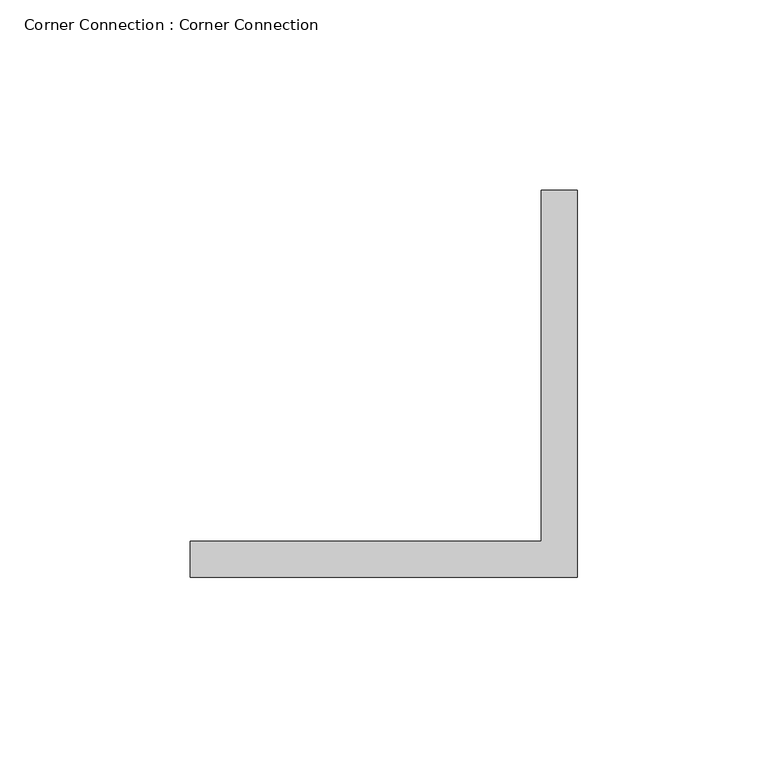
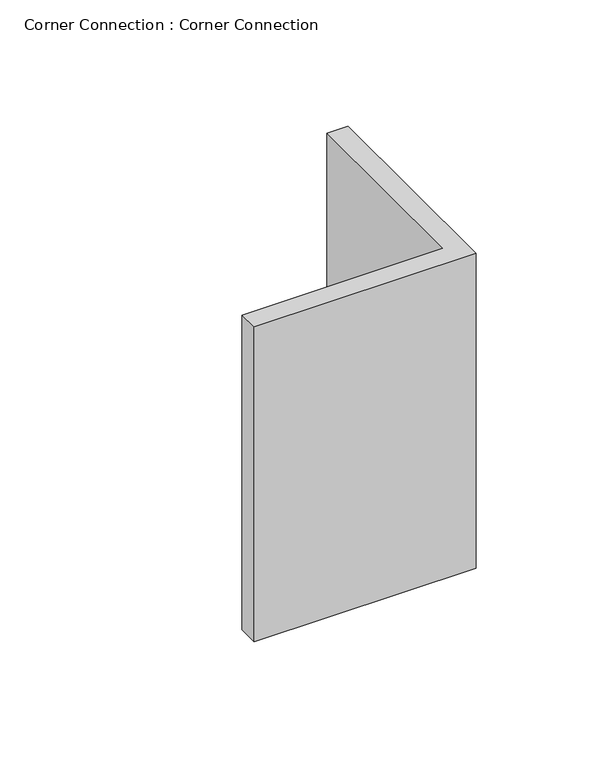
"""IFC4 building model written with IfcOpenShell, lengths in millimetres: fastener geometry, Corner Connection : Corner Connection."""

import ifcopenshell
import ifcopenshell.guid

model = None  # the IFC model being written
_history = None  # IfcOwnerHistory: only IFC2X3 demands one
_inside = {}  # id of a spatial element -> (the spatial element, [elements in it])
_under = {}  # id of a project, library or spatial element -> (it, [spatial elements below it])
_declared = {}  # id of a project -> (the project, [libraries it declares])
_typed = {}  # id of a type object -> (the type object, [elements of that type])
_made_of = {}  # id of a material, layer set ... -> (it, [elements and type objects made of it])


def new_model(schema):
    """Start an empty IFC model of exactly this schema.

    Asked for "IFC4X3", IfcOpenShell would pick the latest addendum, in which some entities
    have other attributes; the version numbers below select the first issue.
    IFC2X3 requires an IfcOwnerHistory on every rooted entity: one is made here for all.
    """
    global model, _history
    if schema == "IFC4X3":
        model = ifcopenshell.file(schema_version=(4, 3, 0, 0))
    else:
        model = ifcopenshell.file(schema=schema)
    _inside.clear()
    _under.clear()
    _declared.clear()
    _typed.clear()
    _made_of.clear()
    _history = None
    if model.schema == "IFC2X3":
        org = make("IfcOrganization", Name="unknown")
        user = make(
            "IfcPersonAndOrganization",
            ThePerson=make("IfcPerson", FamilyName="unknown"),
            TheOrganization=org,
        )
        app = make(
            "IfcApplication",
            ApplicationDeveloper=org,
            Version="unknown",
            ApplicationFullName="unknown",
            ApplicationIdentifier="unknown",
        )
        _history = make(
            "IfcOwnerHistory",
            OwningUser=user,
            OwningApplication=app,
            ChangeAction="ADDED",
            CreationDate=0,
        )
    return model


def make(cls, **values):
    """One entity of the class cls with the attributes given. An attribute that is None is left unset."""
    return model.create_entity(
        cls, **{name: value for name, value in values.items() if value is not None}
    )


def rooted(cls, **values):
    """An entity with a GlobalId (a new one), such as an element, a storey or a relation."""
    return make(cls, GlobalId=ifcopenshell.guid.new(), OwnerHistory=_history, **values)


def si_unit(unit_type, name, prefix=None):
    """IfcSIUnit, for example si_unit("LENGTHUNIT", "METRE", prefix="MILLI")."""
    return make("IfcSIUnit", UnitType=unit_type, Prefix=prefix, Name=name)


def assignment(units):
    """IfcUnitAssignment: the units of a project."""
    return None if units is None else make("IfcUnitAssignment", Units=units)


def point(xyz):
    """IfcCartesianPoint."""
    return None if xyz is None else make("IfcCartesianPoint", Coordinates=xyz)


def direction(xyz):
    """IfcDirection."""
    return None if xyz is None else make("IfcDirection", DirectionRatios=xyz)


def frame(location, z_axis=None, x_axis=None):
    """IfcAxis2Placement3D, a coordinate frame: its origin and axes. An axis left out is left unset."""
    return make(
        "IfcAxis2Placement3D",
        Location=point(location),
        Axis=direction(z_axis),
        RefDirection=direction(x_axis),
    )


def origin():
    """The frame at (0, 0, 0) with its axes left unset."""
    return frame((0.0, 0.0, 0.0))


def origin_with_axes():
    """The frame at (0, 0, 0) with the z axis (0, 0, 1) and the x axis (1, 0, 0) written out."""
    return frame((0.0, 0.0, 0.0), z_axis=(0.0, 0.0, 1.0), x_axis=(1.0, 0.0, 0.0))


def place(relative_to, where):
    """IfcLocalPlacement: puts the frame where relative to a parent placement (None: the world)."""
    return make(
        "IfcLocalPlacement", PlacementRelTo=relative_to, RelativePlacement=where
    )


def context(
    kind, dimensions, precision=None, world=None, true_north=None, identifier=None
):
    """IfcGeometricRepresentationContext, for example the 3D "Model" context."""
    return make(
        "IfcGeometricRepresentationContext",
        ContextIdentifier=identifier,
        ContextType=kind,
        CoordinateSpaceDimension=dimensions,
        Precision=precision,
        WorldCoordinateSystem=world,
        TrueNorth=true_north,
    )


def project(units=None, contexts=None):
    """IfcProject with its units and contexts."""
    return rooted(
        "IfcProject",
        Name="project",
        RepresentationContexts=contexts,
        UnitsInContext=assignment(units),
    )


def spatial(cls, under=None, at=None, **own):
    """A site, building, storey or space (cls), placed at a placement, below another one or the project."""
    s = rooted(cls, ObjectPlacement=at, **own)
    if under is not None:
        _under.setdefault(under.id(), (under, []))[1].append(s)
    return s


def polyline(points):
    """IfcPolyline through the points."""
    return make("IfcPolyline", Points=[point(p) for p in points])


def outline(outer, holes=None, kind="AREA"):
    """IfcArbitraryClosedProfileDef: a profile drawn as a closed curve; with holes, ...WithVoids."""
    if holes is None:
        return make("IfcArbitraryClosedProfileDef", ProfileType=kind, OuterCurve=outer)
    return make(
        "IfcArbitraryProfileDefWithVoids",
        ProfileType=kind,
        OuterCurve=outer,
        InnerCurves=holes,
    )


def extrude(swept, where, along, depth):
    """IfcExtrudedAreaSolid: the profile swept, set in the frame where, extruded along a direction by depth."""
    return make(
        "IfcExtrudedAreaSolid",
        SweptArea=swept,
        Position=where,
        ExtrudedDirection=direction(along),
        Depth=depth,
    )


def shape(context_of_items, identifier, shape_type, items):
    """IfcShapeRepresentation: the items that make up one representation, for example the "Body"."""
    return make(
        "IfcShapeRepresentation",
        ContextOfItems=context_of_items,
        RepresentationIdentifier=identifier,
        RepresentationType=shape_type,
        Items=items,
    )


def source(mapping_origin, context_of_items, identifier, shape_type, items):
    """IfcRepresentationMap: a shape defined once, which mapped items show again and again."""
    return make(
        "IfcRepresentationMap",
        MappingOrigin=mapping_origin,
        MappedRepresentation=shape(context_of_items, identifier, shape_type, items),
    )


def transform(
    local_origin,
    x_axis=None,
    y_axis=None,
    z_axis=None,
    scale=None,
    scale2=None,
    scale3=None,
    uniform=True,
):
    """IfcCartesianTransformationOperator3D, or its non-uniform kind. x_axis, y_axis, z_axis: its Axis1, 2, 3."""
    if uniform:
        return make(
            "IfcCartesianTransformationOperator3D",
            Axis1=direction(x_axis),
            Axis2=direction(y_axis),
            LocalOrigin=point(local_origin),
            Scale=scale,
            Axis3=direction(z_axis),
        )
    return make(
        "IfcCartesianTransformationOperator3DnonUniform",
        Axis1=direction(x_axis),
        Axis2=direction(y_axis),
        LocalOrigin=point(local_origin),
        Scale=scale,
        Axis3=direction(z_axis),
        Scale2=scale2,
        Scale3=scale3,
    )


def mapped(mapping_source, mapping_target):
    """IfcMappedItem: shows the shape of a source again, moved by a transform."""
    return make(
        "IfcMappedItem", MappingSource=mapping_source, MappingTarget=mapping_target
    )


def made_of(thing, what):
    """Note that an element or type object is made of a material, layer set ...; save() writes the relation."""
    if what is not None:
        _made_of.setdefault(what.id(), (what, []))[1].append(thing)
    return thing


def element(
    cls,
    number,
    at=None,
    inside=None,
    cuts=None,
    type_object=None,
    material=None,
    context=None,
    identifier="Body",
    shape_type=None,
    held_by="IfcProductDefinitionShape",
    body=None,
    shapes=None,
    **own,
):
    """One element of the class cls, such as IfcWall. Its Tag is "e" and its number.

    at: its placement. inside: the storey or other place that contains it. cuts: it is an
    opening in that element (IfcRelVoidsElement). A single representation is given by context,
    identifier, shape_type and body (its items); several are given by shapes. held_by: the class
    of the entity that holds the representations. save() writes the other relations.
    """
    e = rooted(cls, Tag="e%d" % number, ObjectPlacement=at, **own)
    if body is not None:
        shapes = [shape(context, identifier, shape_type, body)]
    if shapes is not None:
        e.Representation = make(held_by, Representations=shapes)
    if inside is not None:
        _inside.setdefault(inside.id(), (inside, []))[1].append(e)
    if cuts is not None:
        rooted(
            "IfcRelVoidsElement", RelatingBuildingElement=cuts, RelatedOpeningElement=e
        )
    if type_object is not None:
        _typed.setdefault(type_object.id(), (type_object, []))[1].append(e)
    return made_of(e, material)


def aggregate(whole, parts):
    """IfcRelAggregates: a whole, such as a stair, and the parts it consists of."""
    return rooted("IfcRelAggregates", RelatingObject=whole, RelatedObjects=parts)


def save(model, path):
    """Write the relations noted so far, then the file.

    IfcRelAggregates (storeys below a building ...), IfcRelContainedInSpatialStructure (elements
    in a storey), IfcRelDefinesByType, IfcRelAssociatesMaterial and IfcRelDeclares: one each for
    every whole, place, type object, material and project.
    """
    for whole, parts in _under.values():
        aggregate(whole, parts)
    for where, things in _inside.values():
        rooted(
            "IfcRelContainedInSpatialStructure",
            RelatedElements=things,
            RelatingStructure=where,
        )
    for kind, things in _typed.values():
        rooted("IfcRelDefinesByType", RelatedObjects=things, RelatingType=kind)
    for what, things in _made_of.values():
        rooted("IfcRelAssociatesMaterial", RelatedObjects=things, RelatingMaterial=what)
    for by, libraries in _declared.values():
        rooted("IfcRelDeclares", RelatingContext=by, RelatedDefinitions=libraries)
    model.write(path)


def corner_connection_corner_connection_5270f13b(model_context):
    return source(origin(), model_context, "Body", "SweptSolid", [
        extrude(outline(polyline([(-101.6, 0.0), (-101.6, 9.525), (-9.525, 9.525), (-9.525, 101.6), (0.0, 101.6), (0.0, 0.0), (-101.6, 0.0)])), origin_with_axes(), (0.0, 0.0, 1.0), 152.4),
    ])


if __name__ == "__main__":
    model = new_model("IFC4")
    model_context = context("Model", 3, world=origin())
    ifc_project = project(units=[si_unit("LENGTHUNIT", "METRE", prefix="MILLI")], contexts=[model_context])
    site = spatial("IfcSite", under=ifc_project)
    building = spatial("IfcBuilding", under=site)
    placement = place(None, origin())
    corner_connection_corner_connection_shape = corner_connection_corner_connection_5270f13b(model_context)
    element("IfcFastener", 1, ObjectType="Corner Connection : Corner Connection", at=placement, inside=building, context=model_context, shape_type="MappedRepresentation", body=[
        mapped(corner_connection_corner_connection_shape, transform((0.0, 0.0, 0.0), x_axis=(1.0, 0.0, 0.0), y_axis=(0.0, 1.0, 0.0), z_axis=(0.0, 0.0, 1.0))),
    ])
    save(model, "model.ifc")

# Revit data of these elements
# Type "Corner Connection : Corner Connection"
#   MATERIAL = Galvanized Steel
# Element 1 (IfcFastener, "Corner Connection : Corner Connection")
#   Materials on its faces: "Galvanized Steel"
# Materials
#   "Galvanized Steel": class "Generic", colour RGB 232 232 232, transparency 0, Description = "Acoustic Ceiling Tile 24 x 24", Cost = 0
